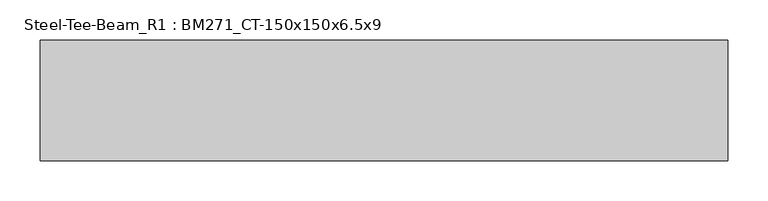
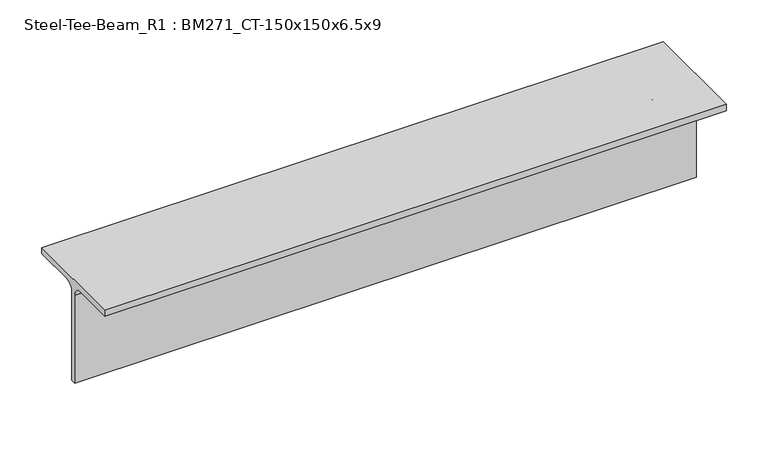
"""IFC4 building model written with IfcOpenShell, lengths in millimetres: member geometry, Steel-Tee-Beam_R1 : BM271_CT-150x150x6.5x9."""

from ifc_helpers import new_model, si_unit, point, frame, frame_2d, origin, place, context, project, spatial, polyline, circle_curve, trimmed, segment, composite_curve, outline, extrude, source, transform, mapped, element, save


def steel_tee_beam_r1_bm271_ct_150x150x6_5x9_59417580(model_context):
    return source(origin(), model_context, "Body", "SweptSolid", [
        extrude(outline(composite_curve([segment(polyline([(-75.0, 75.0), (75.0, 75.0), (75.0, 66.0), (16.25, 66.0)]), True, "CONTINUOUS"), segment(trimmed(circle_curve(frame_2d((16.25, 53.0)), 13.0), [point((16.25, 66.0))], [point((3.25, 53.0))], True, "CARTESIAN"), True, "CONTINUOUS"), segment(polyline([(3.25, 53.0), (3.25, -75.0), (-3.25, -75.0), (-3.25, 53.0)]), True, "CONTINUOUS"), segment(trimmed(circle_curve(frame_2d((-16.25, 53.0)), 13.0), [point((-3.25, 53.0))], [point((-16.25, 66.0))], True, "CARTESIAN"), True, "CONTINUOUS"), segment(polyline([(-16.25, 66.0), (-75.0, 66.0), (-75.0, 75.0)]), True, "CONTINUOUS")], self_intersect=False)), frame((-356.1687518, 0.0, 0.0), z_axis=(1.0, 0.0, 0.0), x_axis=(0.0, 1.0, 0.0)), (0.0, 0.0, 1.0), 856.1687518),
    ])


if __name__ == "__main__":
    model = new_model("IFC4")
    model_context = context("Model", 3, world=origin())
    ifc_project = project(units=[si_unit("LENGTHUNIT", "METRE", prefix="MILLI")], contexts=[model_context])
    site = spatial("IfcSite", under=ifc_project)
    building = spatial("IfcBuilding", under=site)
    placement = place(None, origin())
    steel_tee_beam_r1_bm271_ct_150x150x6_5x9_shape = steel_tee_beam_r1_bm271_ct_150x150x6_5x9_59417580(model_context)
    element("IfcMember", 1, ObjectType="Steel-Tee-Beam_R1 : BM271_CT-150x150x6.5x9", at=placement, inside=building, context=model_context, shape_type="MappedRepresentation", body=[
        mapped(steel_tee_beam_r1_bm271_ct_150x150x6_5x9_shape, transform((0.0, 0.0, 0.0), x_axis=(1.0, 0.0, 0.0), y_axis=(0.0, 1.0, 0.0), z_axis=(0.0, 0.0, 1.0))),
    ])
    save(model, "model.ifc")

# Revit data of these elements
# Type "Steel-Tee-Beam_R1 : BM271_CT-150x150x6.5x9"
#   Keynote = "CT-150x150x6.5x9"
#   Surface Area = 0.588841 m²/m
#   Section Area = 23.3904 cm²
#   Mass per Unit Length = 18.3614 kg/m
#   Length [instance default] = 1.5240 m
#   bf = 0.1500 m
#   d = 0.1500 m
#   k = 0.0220 m
#   r = 0.0130 m
#   tf = 0.0090 m
#   tw = 0.0065 m
#   hec_material4 [instance default] = none
#   hec_material3 [instance default] = none
#   hec_material2 [instance default] = none
#   hec_material1 [instance default] = none
#   Structural Material [instance default] = Steel, 45-345
#   Assembly Code = ""
# Element 1 (IfcMember, "Steel-Tee-Beam_R1 : BM271_CT-150x150x6.5x9")
#   Structural Material = none
# Materials
#   "Steel, 45-345": class "Metal", colour RGB 189 187 185, transparency 0, Description = "Steel 345 MPa", Cost = 0
